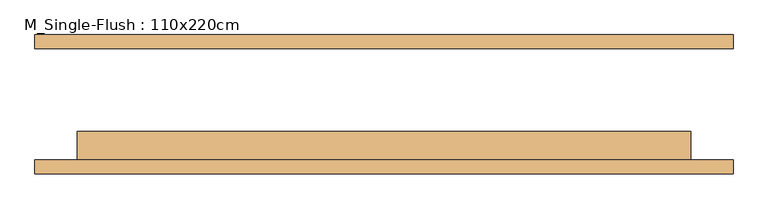
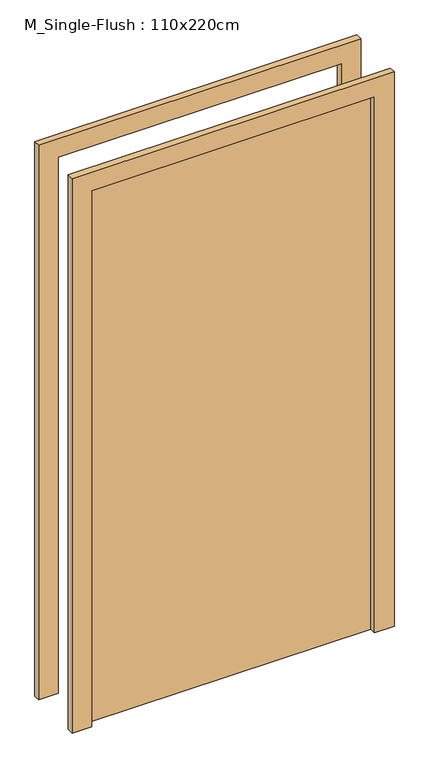
"""IFC4 building model written with IfcOpenShell, lengths in millimetres: door geometry, M_Single-Flush : 110x220cm."""

from ifc_helpers import new_model, si_unit, frame, origin, origin_with_axes, place, context, project, spatial, polyline, outline, extrude, source, transform, mapped, element, save


def m_single_flush_110x220cm_1551c729(model_context):
    return source(origin(), model_context, "Body", "SweptSolid", [
        extrude(outline(polyline([(2276.0, -626.0), (0.0, -626.0), (0.0, -550.0), (2200.0, -550.0), (2200.0, 550.0), (0.0, 550.0), (0.0, 626.0), (2276.0, 626.0), (2276.0, -626.0)])), frame((0.0, -125.0, 0.0), z_axis=(0.0, 1.0, 0.0), x_axis=(0.0, 0.0, 1.0)), (0.0, 0.0, 1.0), 25.0),
        extrude(outline(polyline([(2276.0, 626.0), (2276.0, -626.0), (0.0, -626.0), (0.0, -550.0), (2200.0, -550.0), (2200.0, 550.0), (0.0, 550.0), (0.0, 626.0), (2276.0, 626.0)])), frame((0.0, 100.0, 0.0), z_axis=(0.0, 1.0, 0.0), x_axis=(0.0, 0.0, 1.0)), (0.0, 0.0, 1.0), 25.0),
        extrude(outline(polyline([(550.0, -49.0), (550.0, -100.0), (-550.0, -100.0), (-550.0, -49.0), (550.0, -49.0)])), origin_with_axes(), (0.0, 0.0, 1.0), 2200.0),
    ])


if __name__ == "__main__":
    model = new_model("IFC4")
    model_context = context("Model", 3, world=origin())
    ifc_project = project(units=[si_unit("LENGTHUNIT", "METRE", prefix="MILLI")], contexts=[model_context])
    site = spatial("IfcSite", under=ifc_project)
    building = spatial("IfcBuilding", under=site)
    placement = place(None, origin())
    m_single_flush_110x220cm_shape = m_single_flush_110x220cm_1551c729(model_context)
    element("IfcDoor", 1, ObjectType="M_Single-Flush : 110x220cm", at=placement, inside=building, context=model_context, shape_type="MappedRepresentation", body=[
        mapped(m_single_flush_110x220cm_shape, transform((0.0, 0.0, 0.0), x_axis=(1.0, 0.0, 0.0), y_axis=(0.0, 1.0, 0.0), z_axis=(0.0, 0.0, 1.0))),
    ])
    save(model, "model.ifc")

# Revit data of these elements
# Type "M_Single-Flush : 110x220cm"
#   Type Mark = "45"
#   Construction Type Id = "MDOOR"
#   Analytic Construction = "Metal"
#   Thickness = 5.10 cm
#   Heat Transfer Coefficient (U) = 3.7021 W/(m²·K)
#   Height = 220.00 cm
#   Trim Projection Ext = 2.50 cm
#   Trim Projection Int = 2.50 cm
#   Trim Width = 7.60 cm
#   Width = 110.00 cm
#   Define Thermal Properties by = 1
#   Door Material = Door - Panel
#   Frame Material = Door - Frame
#   Visual Light Transmittance = 0
#   Solar Heat Gain Coefficient = 0
#   Function = (empty or 0)
#   Wall Closure = (empty or 0)
# Element 1 (IfcDoor, "M_Single-Flush : 110x220cm")
#   Materials on its faces: "Door - Frame", "Door - Panel"
# Materials
#   "Door - Panel": class "Wood", colour RGB 210 159 95, transparency 0, Cost = 0
#   "Door - Frame": class "Miscellaneous", colour RGB 118 70 51, transparency 0, Cost = 0
